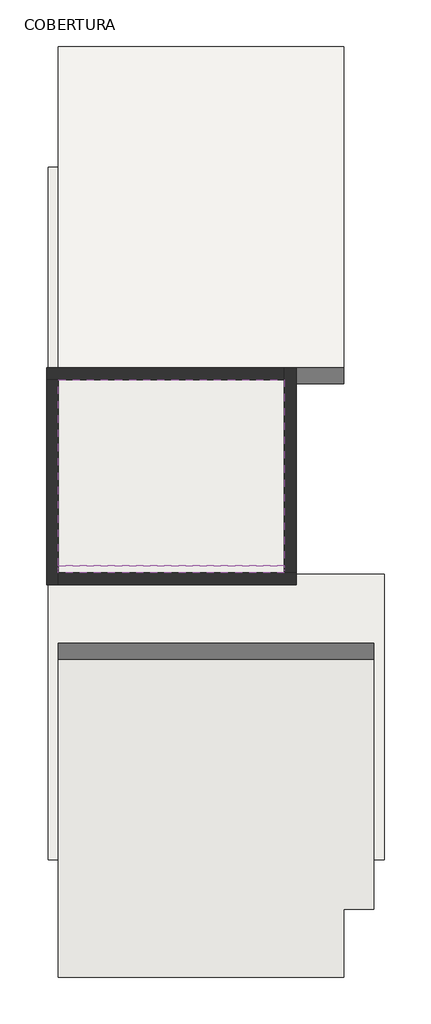
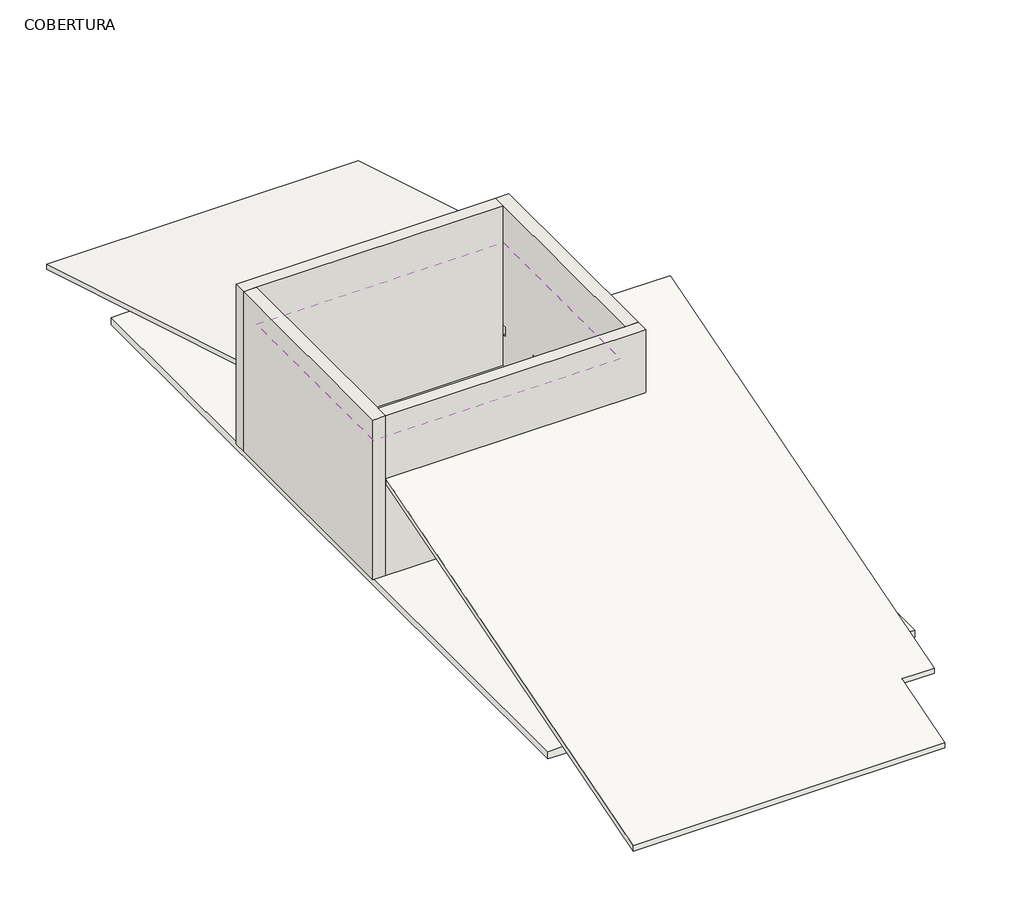
# One storey: 4 walls, 3 roofs, 1 pipe segment, 1 slab.
"""IFC4 building model written with IfcOpenShell, lengths in millimetres."""

from ifc_helpers import new_model, si_unit, frame, origin, place, context, project, spatial, polyline, outline, extrude, faceted_brep, element, save

model = new_model("IFC4")

# Units and contexts
model_context = context("Model", 3, world=origin())
ifc_project = project(units=[si_unit("LENGTHUNIT", "METRE", prefix="MILLI")], contexts=[model_context])

# Site, building, storey
site = spatial("IfcSite", under=ifc_project)
building = spatial("IfcBuilding", under=site)
storey = spatial("IfcBuildingStorey", under=building, Name="COBERTURA", Elevation=6160.0)

# Pipe segment
placement = place(None, origin())
element("IfcPipeSegment", 1, ObjectType=".CALHA 12.5 cm", at=placement, inside=storey, context=model_context, shape_type="SweptSolid", body=[
    extrude(outline(polyline([(-2115.2624019, 8115.4867724), (-2189.4624019, 8115.4867724), (-2227.5624019, 8214.999005), (-2240.2624019, 8214.999005), (-2240.2624019, 8227.699005), (-2227.5624019, 8227.699005), (-2227.5624019, 8224.524005), (-2237.0874019, 8224.524005), (-2237.0874019, 8218.174005), (-2225.2001046, 8218.174005), (-2187.1001046, 8118.6617724), (-2118.4374019, 8118.6617724), (-2118.4374019, 8240.399005), (-2115.2624019, 8240.399005), (-2115.2624019, 8115.4867724)])), frame((-2574.4431325, 0.0, 0.0), z_axis=(1.0, 0.0, 0.0), x_axis=(0.0, 1.0, 0.0)), (0.0, 0.0, 1.0), 3800.0),
])

# Roofs
element("IfcRoof", 2, ObjectType="TELHA METÁLICA", at=placement, inside=storey, context=model_context, shape_type="SweptSolid", body=[
    extrude(outline(polyline([(-2115.2624019, 8240.399005), (1009.7375981, 8552.899005), (1009.7375981, 8472.5), (-2115.2624019, 8160.0), (-2115.2624019, 8240.399005)])), frame((-2574.4431325, 0.0, 0.0), z_axis=(1.0, 0.0, 0.0), x_axis=(0.0, 1.0, 0.0)), (0.0, 0.0, 1.0), 3800.0),
])
element("IfcRoof", 3, ObjectType=".TELHA CERÂMICA", at=placement, inside=storey, context=model_context, shape_type="Brep", body=[
    faceted_brep([(1425.5568675, 1209.7375981, 7280.0), (-2574.4431325, 1209.7375981, 7280.0), (-2574.4431325, 6609.7375981, 5660.0), (2225.5568675, 6609.7375981, 5660.0), (2225.5568675, 409.7375981, 7520.0), (1425.5568675, 409.7375981, 7520.0), (-2574.4431325, 1209.7375981, 7363.5224521), (1425.5568675, 1209.7375981, 7363.5224521), (1425.5568675, 409.7375981, 7603.5224521), (2225.5568675, 409.7375981, 7603.5224521), (2225.5568675, 6609.7375981, 5743.5224521), (-2574.4431325, 6609.7375981, 5743.5224521)], [[[0, 1, 2, 3, 4, 5]], [[6, 7, 8, 9, 10, 11]], [[2, 11, 10, 3]], [[7, 6, 1, 0]], [[6, 11, 2, 1]], [[10, 9, 4, 3]], [[8, 7, 0, 5]], [[9, 8, 5, 4]]]),
])
element("IfcRoof", 4, ObjectType=".TELHA CERÂMICA", at=placement, inside=storey, context=model_context, shape_type="Brep", body=[
    faceted_brep([(-2574.4431325, -2440.2624019, 7655.0), (1425.5568675, -2440.2624019, 7655.0), (1425.5568675, -840.2624019, 8135.0), (2725.5568675, -840.2624019, 8135.0), (2725.5568675, -7890.2624019, 6020.0), (2225.5568675, -7890.2624019, 6020.0), (2225.5568675, -9040.2624019, 5675.0), (-2574.4431325, -9040.2624019, 5675.0), (1425.5568675, -2440.2624019, 7738.5224521), (-2574.4431325, -2440.2624019, 7738.5224521), (-2574.4431325, -9040.2624019, 5758.5224521), (2225.5568675, -9040.2624019, 5758.5224521), (2225.5568675, -7890.2624019, 6103.5224521), (2725.5568675, -7890.2624019, 6103.5224521), (2725.5568675, -840.2624019, 8218.5224521), (1425.5568675, -840.2624019, 8218.5224521)], [[[0, 1, 2, 3, 4, 5, 6, 7]], [[8, 9, 10, 11, 12, 13, 14, 15]], [[6, 11, 10, 7]], [[9, 8, 1, 0]], [[10, 9, 0, 7]], [[14, 13, 4, 3]], [[15, 14, 3, 2]], [[8, 15, 2, 1]], [[12, 11, 6, 5]], [[13, 12, 5, 4]]]),
])

# Slab
element("IfcSlab", 5, ObjectType=".EST. LAJE 12 cm - CONCRETO", at=placement, inside=storey, context=model_context, shape_type="Brep", body=[
    faceted_brep([(1400.5568675, 4584.7375981, 6040.0), (1400.5568675, 1134.7375981, 6040.0), (1400.5568675, -240.6624019, 6040.0), (1400.5568675, -2265.2624019, 6040.0), (1425.5568675, -2265.2624019, 6040.0), (2900.5568675, -2265.2624019, 6040.0), (2900.5568675, -3815.2624019, 6040.0), (2900.5568675, -7065.2624019, 6040.0), (2725.5568675, -7065.2624019, 6040.0), (-2574.4431325, -7065.2624019, 6040.0), (-2749.4431325, -7065.2624019, 6040.0), (-2749.4431325, 4584.7375981, 6040.0), (-2574.4431325, 4584.7375981, 6040.0), (1225.5568675, 4584.7375981, 6040.0), (1400.5568675, 4584.7375981, 6160.0), (1225.5568675, 4584.7375981, 6160.0), (-2574.4431325, 4584.7375981, 6160.0), (-2749.4431325, 4584.7375981, 6160.0), (-2749.4431325, 1209.7375981, 6160.0), (-2749.4431325, -2440.2624019, 6160.0), (-2749.4431325, -7065.2624019, 6160.0), (-2574.4431325, -7065.2624019, 6160.0), (2725.5568675, -7065.2624019, 6160.0), (2900.5568675, -7065.2624019, 6160.0), (2900.5568675, -3815.2624019, 6160.0), (2900.5568675, -2265.2624019, 6160.0), (1425.5568675, -2265.2624019, 6160.0), (1400.5568675, -2265.2624019, 6160.0), (1400.5568675, -240.6624019, 6160.0), (1400.5568675, 1134.7375981, 6160.0), (1400.5568675, 1209.7375981, 6160.0)], [[[0, 1, 2, 3, 4, 5, 6, 7, 8, 9, 10, 11, 12, 13]], [[14, 15, 16, 17, 18, 19, 20, 21, 22, 23, 24, 25, 26, 27, 28, 29, 30]], [[3, 2, 1, 0, 14, 30, 29, 28, 27]], [[5, 4, 3, 27, 26, 25]], [[7, 6, 5, 25, 24, 23]], [[10, 9, 8, 7, 23, 22, 21, 20]], [[11, 10, 20, 19, 18, 17]], [[0, 13, 12, 11, 17, 16, 15, 14]]]),
])

# Walls
element("IfcWall", 6, ObjectType=".EXT. PAREDE 20 cm - PINTURA/PINTURA", at=placement, inside=storey, context=model_context, shape_type="Brep", body=[
    faceted_brep([(-2774.4431325, 1009.7375981, 8760.0), (-2774.4431325, 1009.7375981, 6160.0), (-2574.4431325, 1009.7375981, 6160.0), (1225.5568675, 1009.7375981, 6160.0), (1225.5568675, 1009.7375981, 6660.0), (1225.5568675, 1009.7375981, 6810.0), (1225.5568675, 1009.7375981, 6830.0), (1225.5568675, 1009.7375981, 8760.0), (-2574.4431325, 1009.7375981, 8760.0), (-2774.4431325, 1209.7375981, 6160.0), (-2774.4431325, 1209.7375981, 7542.5413482), (-2774.4431325, 1209.7375981, 8760.0), (1225.5568675, 1209.7375981, 8760.0), (1225.5568675, 1209.7375981, 6160.0), (-2574.4431325, 1209.7375981, 6160.0), (1225.5568675, 1184.7375981, 6160.0), (-2774.4431325, 1184.7375981, 6160.0)], [[[0, 1, 2, 3, 4, 5, 6, 7, 8]], [[9, 10, 11, 12, 13, 14]], [[0, 8, 7, 12, 11]], [[7, 6, 5, 4, 3, 15, 13, 12]], [[3, 2, 1, 16, 15]], [[16, 9, 14, 13, 15]], [[0, 11, 10, 9, 16, 1]]]),
])
element("IfcWall", 7, ObjectType=".EXT. PAREDE 20 cm - PINTURA/PINTURA", at=placement, inside=storey, context=model_context, shape_type="Brep", body=[
    faceted_brep([(-2574.4431325, -2440.2624019, 6160.0), (-2574.4431325, -2240.2624019, 6160.0), (-2574.4431325, 1009.7375981, 6160.0), (-2574.4431325, 1009.7375981, 6660.0), (-2574.4431325, 959.7375981, 6660.0), (-2574.4431325, 959.7375981, 6810.0), (-2574.4431325, 1009.7375981, 6810.0), (-2574.4431325, 1009.7375981, 6830.0), (-2574.4431325, 1009.7375981, 8760.0), (-2574.4431325, -2240.2624019, 8760.0), (-2574.4431325, -2440.2624019, 8760.0), (-2574.4431325, -2440.2624019, 7917.4966495), (-2574.4431325, -1440.2624019, 6810.0), (-2574.4431325, -1390.2624019, 6810.0), (-2574.4431325, -1390.2624019, 6660.0), (-2574.4431325, -1440.2624019, 6660.0), (-2574.4431325, -640.2624019, 6810.0), (-2574.4431325, -590.2624019, 6810.0), (-2574.4431325, -590.2624019, 6660.0), (-2574.4431325, -640.2624019, 6660.0), (-2574.4431325, 159.7375981, 6810.0), (-2574.4431325, 209.7375981, 6810.0), (-2574.4431325, 209.7375981, 6660.0), (-2574.4431325, 159.7375981, 6660.0), (-2574.4431325, -2240.2624019, 6810.0), (-2574.4431325, -2190.2624019, 6810.0), (-2574.4431325, -2190.2624019, 6660.0), (-2574.4431325, -2240.2624019, 6660.0), (-2774.4431325, -2440.2624019, 8760.0), (-2774.4431325, 1009.7375981, 8760.0), (-2774.4431325, 1009.7375981, 6160.0), (-2774.4431325, -2440.2624019, 6160.0), (-2774.4431325, -2440.2624019, 7917.4966495), (-2749.4431325, -2440.2624019, 6160.0), (-2749.4431325, 1009.7375981, 6160.0), (-2724.4431325, 1009.7375981, 6810.0), (-2724.4431325, 1009.7375981, 6660.0), (-2724.4431325, -1440.2624019, 6810.0), (-2724.4431325, -1390.2624019, 6810.0), (-2724.4431325, -1390.2624019, 6660.0), (-2724.4431325, -1440.2624019, 6660.0), (-2724.4431325, -640.2624019, 6810.0), (-2724.4431325, -590.2624019, 6810.0), (-2724.4431325, -590.2624019, 6660.0), (-2724.4431325, -640.2624019, 6660.0), (-2724.4431325, 159.7375981, 6810.0), (-2724.4431325, 209.7375981, 6810.0), (-2724.4431325, 209.7375981, 6660.0), (-2724.4431325, 159.7375981, 6660.0), (-2724.4431325, -2240.2624019, 6810.0), (-2724.4431325, -2190.2624019, 6810.0), (-2724.4431325, -2190.2624019, 6660.0), (-2724.4431325, -2240.2624019, 6660.0), (-2724.4431325, 959.7375981, 6810.0), (-2724.4431325, 959.7375981, 6660.0)], [[[0, 1, 2, 3, 4, 5, 6, 7, 8, 9, 10, 11], [12, 13, 14, 15], [16, 17, 18, 19], [20, 21, 22, 23], [24, 25, 26, 27]], [[28, 29, 30, 31, 32]], [[10, 9, 8, 29, 28]], [[2, 1, 0, 33, 34]], [[33, 31, 30, 34]], [[10, 28, 32, 31, 33, 0, 11]], [[29, 8, 7, 6, 35, 36, 3, 2, 34, 30]], [[37, 38, 13, 12]], [[39, 40, 15, 14]], [[38, 39, 14, 13]], [[38, 37, 40, 39]], [[40, 37, 12, 15]], [[41, 42, 17, 16]], [[43, 44, 19, 18]], [[42, 43, 18, 17]], [[42, 41, 44, 43]], [[44, 41, 16, 19]], [[45, 46, 21, 20]], [[47, 48, 23, 22]], [[46, 47, 22, 21]], [[46, 45, 48, 47]], [[48, 45, 20, 23]], [[49, 50, 25, 24]], [[51, 52, 27, 26]], [[50, 51, 26, 25]], [[50, 49, 52, 51]], [[52, 49, 24, 27]], [[53, 35, 6, 5]], [[36, 54, 4, 3]], [[35, 53, 54, 36]], [[54, 53, 5, 4]]]),
])
element("IfcWall", 8, ObjectType=".EXT. PAREDE 20 cm - PINTURA/PINTURA", at=placement, inside=storey, context=model_context, shape_type="Brep", body=[
    faceted_brep([(1425.5568675, -2240.2624019, 6160.0), (1225.5568675, -2240.2624019, 6160.0), (-2574.4431325, -2240.2624019, 6160.0), (-2574.4431325, -2240.2624019, 6660.0), (-2574.4431325, -2240.2624019, 6810.0), (-2574.4431325, -2240.2624019, 6830.0), (-2574.4431325, -2240.2624019, 8760.0), (1225.5568675, -2240.2624019, 8760.0), (1425.5568675, -2240.2624019, 8760.0), (1425.5568675, -2440.2624019, 6160.0), (1425.5568675, -2440.2624019, 8760.0), (-2574.4431325, -2440.2624019, 8760.0), (-2574.4431325, -2440.2624019, 6160.0), (1425.5568675, -2415.2624019, 6160.0), (-2574.4431325, -2415.2624019, 6160.0)], [[[0, 1, 2, 3, 4, 5, 6, 7, 8]], [[9, 10, 11, 12]], [[8, 7, 6, 11, 10]], [[0, 8, 10, 9, 13]], [[2, 1, 0, 13, 14]], [[13, 9, 12, 14]], [[2, 14, 12, 11, 6, 5, 4, 3]]]),
])
element("IfcWall", 9, ObjectType=".EXT. PAREDE 20 cm - PINTURA/PINTURA", at=placement, inside=storey, context=model_context, shape_type="Brep", body=[
    faceted_brep([(1225.5568675, 1209.7375981, 6160.0), (1225.5568675, 1009.7375981, 6160.0), (1225.5568675, -2240.2624019, 6160.0), (1225.5568675, -2240.2624019, 6660.0), (1225.5568675, -2190.2624019, 6660.0), (1225.5568675, -2190.2624019, 6810.0), (1225.5568675, -2240.2624019, 6810.0), (1225.5568675, -2240.2624019, 6830.0), (1225.5568675, -2240.2624019, 8760.0), (1225.5568675, 1009.7375981, 8760.0), (1225.5568675, 1209.7375981, 8760.0), (1225.5568675, 1209.7375981, 7280.0), (1225.5568675, -1390.2624019, 6810.0), (1225.5568675, -1440.2624019, 6810.0), (1225.5568675, -1440.2624019, 6660.0), (1225.5568675, -1390.2624019, 6660.0), (1225.5568675, -590.2624019, 6810.0), (1225.5568675, -640.2624019, 6810.0), (1225.5568675, -640.2624019, 6660.0), (1225.5568675, -590.2624019, 6660.0), (1225.5568675, 209.7375981, 6810.0), (1225.5568675, 159.7375981, 6810.0), (1225.5568675, 159.7375981, 6660.0), (1225.5568675, 209.7375981, 6660.0), (1225.5568675, 1009.7375981, 6810.0), (1225.5568675, 959.7375981, 6810.0), (1225.5568675, 959.7375981, 6660.0), (1225.5568675, 1009.7375981, 6660.0), (1425.5568675, 1209.7375981, 8760.0), (1425.5568675, -2240.2624019, 8760.0), (1425.5568675, -2240.2624019, 6160.0), (1425.5568675, -240.6624019, 6160.0), (1425.5568675, 1134.7375981, 6160.0), (1425.5568675, 1209.7375981, 6160.0), (1425.5568675, 1209.7375981, 7280.0), (1400.5568675, 1209.7375981, 6160.0), (1375.5568675, -2240.2624019, 6810.0), (1375.5568675, -2240.2624019, 6660.0), (1400.5568675, -2240.2624019, 6160.0), (1375.5568675, -1390.2624019, 6810.0), (1375.5568675, -1440.2624019, 6810.0), (1375.5568675, -1440.2624019, 6660.0), (1375.5568675, -1390.2624019, 6660.0), (1375.5568675, -590.2624019, 6810.0), (1375.5568675, -640.2624019, 6810.0), (1375.5568675, -640.2624019, 6660.0), (1375.5568675, -590.2624019, 6660.0), (1375.5568675, 209.7375981, 6810.0), (1375.5568675, 159.7375981, 6810.0), (1375.5568675, 159.7375981, 6660.0), (1375.5568675, 209.7375981, 6660.0), (1375.5568675, -2190.2624019, 6810.0), (1375.5568675, -2190.2624019, 6660.0), (1375.5568675, 1009.7375981, 6810.0), (1375.5568675, 959.7375981, 6810.0), (1375.5568675, 959.7375981, 6660.0), (1375.5568675, 1009.7375981, 6660.0)], [[[0, 1, 2, 3, 4, 5, 6, 7, 8, 9, 10, 11], [12, 13, 14, 15], [16, 17, 18, 19], [20, 21, 22, 23], [24, 25, 26, 27]], [[28, 29, 30, 31, 32, 33, 34]], [[10, 9, 8, 29, 28]], [[0, 11, 10, 28, 34, 33, 35]], [[30, 29, 8, 7, 6, 36, 37, 3, 2, 38]], [[2, 1, 0, 35, 38]], [[35, 33, 32, 31, 30, 38]], [[39, 40, 13, 12]], [[41, 42, 15, 14]], [[40, 39, 42, 41]], [[42, 39, 12, 15]], [[40, 41, 14, 13]], [[43, 44, 17, 16]], [[45, 46, 19, 18]], [[44, 43, 46, 45]], [[46, 43, 16, 19]], [[44, 45, 18, 17]], [[47, 48, 21, 20]], [[49, 50, 23, 22]], [[48, 47, 50, 49]], [[50, 47, 20, 23]], [[48, 49, 22, 21]], [[51, 36, 6, 5]], [[37, 52, 4, 3]], [[36, 51, 52, 37]], [[52, 51, 5, 4]], [[53, 54, 25, 24]], [[55, 56, 27, 26]], [[54, 53, 56, 55]], [[56, 53, 24, 27]], [[54, 55, 26, 25]]]),
])

save(model, "model.ifc")

# Revit data of these elements
# Project information
#   Data de emissão do projeto = "Data de emissão"
#   Status do projeto = "Status do projeto"
# Type "TELHA METÁLICA"
#   Layers, outside or top first: 0.08 m ".TELHA METÁLICA" (function 1)
# Type ".TELHA CERÂMICA"
#   Layers, outside or top first: 0.08 m ".TELHAS" (function 1)
# Type ".EST. LAJE 12 cm - CONCRETO"
#   Function = 0
#   Layers, outside or top first: 0.12 m ".CONCRETO ESTRUTURAL" (function 1)
# Type ".EXT. PAREDE 20 cm - PINTURA/PINTURA"
#   Layers, outside or top first: 0.025 m ".ARGAMASSA + PINTURA BRANCA" (function 5); 0.15 m ".ALVENARIA" (function 1); 0.025 m ".ARGAMASSA + PINTURA BRANCA" (function 5)
# Element 1 (IfcPipeSegment, ".CALHA 12.5 cm")
#   Phase Created = Construção nova
#   Materials on its faces: ".ALUMÍNIO"
# Element 2 (IfcRoof, "TELHA METÁLICA")
#   built-in parameter 1001705 = 28.0607 (stored number, unit not read)
#   built-in parameter 1001710 = 33615
#   Phase Created = Construção nova
#   Materials on its faces: ".TELHA METÁLICA"
# Element 3 (IfcRoof, ".TELHA CERÂMICA")
#   built-in parameter 1001705 = 24.9459 (stored number, unit not read)
#   built-in parameter 1001701 = -1.64042 (stored number, unit not read)
#   built-in parameter 1001710 = 33615
#   Phase Created = Construção nova
#   Materials on its faces: ".TELHAS"
# Element 4 (IfcRoof, ".TELHA CERÂMICA")
#   built-in parameter 1001705 = 26.9637 (stored number, unit not read)
#   built-in parameter 1001701 = -1.59121 (stored number, unit not read)
#   built-in parameter 1001710 = 33615
#   Phase Created = Construção nova
#   Materials on its faces: ".TELHAS"
# Element 5 (IfcSlab, ".EST. LAJE 12 cm - CONCRETO")
#   built-in parameter 1001955 = 1.5708 (stored number, unit not read)
#   Height Offset From Level = 0.00 m
#   Phase Created = Construção nova
#   Materials on its faces: ".CONCRETO ESTRUTURAL"
# Elements 6, 7, 8, 9 (IfcWall, ".EXT. PAREDE 20 cm - PINTURA/PINTURA")
#   Top Offset = 2.88 m
#   Base Offset = 0.00 m
#   Unconnected Height = 2.60 m
#   wall height = 2.60 m
#   Phase Created = Construção nova
#   Base Constraint = COBERTURA
#   Materials on its faces: ".ARGAMASSA + PINTURA BRANCA"
# Materials
#   ".TELHA METÁLICA": class "Genérico", colour RGB 120 120 120, transparency 0, Cost = 0
#   ".TELHAS": class "Genérico", colour RGB 134 55 46, transparency 0, Cost = 0
#   ".CONCRETO ESTRUTURAL": class "Genérico", colour RGB 155 155 155, transparency 0, Description = "Material de telhado betuminoso", Cost = 0
#   ".ARGAMASSA + PINTURA BRANCA": class "Genérico", colour RGB 255 255 255, transparency 0, Cost = 0
#   ".ALVENARIA": class "Alvenaria", colour RGB 192 192 192, transparency 0, Comments = "m²", Description = "Alvenaria em tijolo comum, bloco cerâmico ou bloco de concreto", Cost = 0
#   ".ALUMÍNIO": class "CC_METAIS", colour RGB 244 244 244, transparency 0, Description = "Material alumínio", Cost = 0
